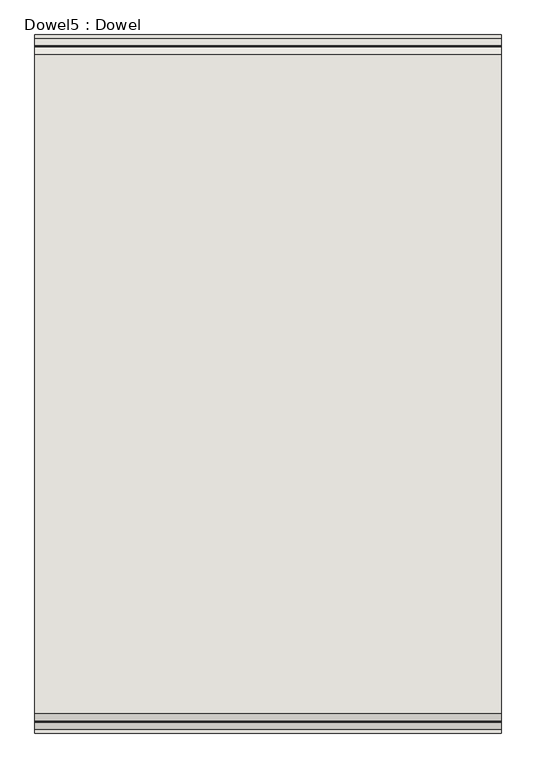
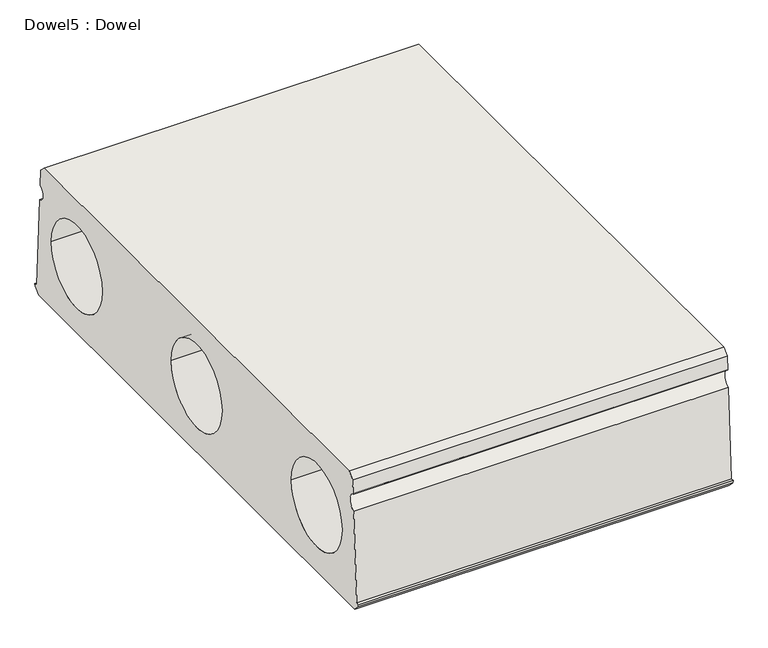
"""IFC4 building model written with IfcOpenShell, lengths in millimetres: wall geometry, Dowel5 : Dowel."""

from ifc_helpers import new_model, si_unit, point, frame, frame_2d, origin, place, context, project, spatial, polyline, circle_curve, trimmed, segment, composite_curve, outline, extrude, source, transform, mapped, element, save


def dowel5_dowel_d00426a0(model_context):
    return source(origin(), model_context, "Body", "SweptSolid", [
        extrude(outline(composite_curve([segment(polyline([(-652.2998095, 2540.0), (494.5752653, 2540.0), (507.2752399, 2527.3000254), (509.1208332, 2491.0485676)]), True, "CONTINUOUS"), segment(trimmed(circle_curve(frame_2d((514.6427832, 2474.6224141)), 17.3294677), [point((509.1208332, 2491.0485676))], [point((511.3260506, 2457.6133067))], True, "CARTESIAN"), True, "CONTINUOUS"), segment(polyline([(511.3260506, 2457.6133067), (523.1502399, 2254.199962), (529.1502279, 2254.199962), (528.4502293, 2248.199974), (515.4502553, 2235.2), (-673.1747995, 2235.2), (-686.1747735, 2248.199974), (-686.8747721, 2254.199962), (-680.8747841, 2254.199962), (-669.0505948, 2457.6133067)]), True, "CONTINUOUS"), segment(trimmed(circle_curve(frame_2d((-675.4772325, 2477.01932)), 20.4424809), [point((-669.0505948, 2457.6133067))], [point((-666.8453774, 2495.55))], True, "CARTESIAN"), True, "CONTINUOUS"), segment(polyline([(-666.8453774, 2495.55), (-664.9997841, 2527.3000254), (-652.2998095, 2540.0)]), True, "CONTINUOUS")], self_intersect=False), holes=[composite_curve([segment(trimmed(circle_curve(frame_2d((-529.7122721, 2387.6)), 95.25), [point((-624.9622721, 2387.6))], [point((-434.4622721, 2387.6))], True, "CARTESIAN"), True, "CONTINUOUS"), segment(trimmed(circle_curve(frame_2d((-529.7122721, 2387.6)), 95.25), [point((-434.4622721, 2387.6))], [point((-624.9622721, 2387.6))], True, "CARTESIAN"), True, "CONTINUOUS")], self_intersect=False), composite_curve([segment(trimmed(circle_curve(frame_2d((-78.8622721, 2387.6)), 95.25), [point((-174.1122721, 2387.6))], [point((16.3877279, 2387.6))], True, "CARTESIAN"), True, "CONTINUOUS"), segment(trimmed(circle_curve(frame_2d((-78.8622721, 2387.6)), 95.25), [point((16.3877279, 2387.6))], [point((-174.1122721, 2387.6))], True, "CARTESIAN"), True, "CONTINUOUS")], self_intersect=False), composite_curve([segment(trimmed(circle_curve(frame_2d((371.9877279, 2387.6)), 95.25), [point((276.7377279, 2387.6))], [point((467.2377279, 2387.6))], True, "CARTESIAN"), True, "CONTINUOUS"), segment(trimmed(circle_curve(frame_2d((371.9877279, 2387.6)), 95.25), [point((467.2377279, 2387.6))], [point((276.7377279, 2387.6))], True, "CARTESIAN"), True, "CONTINUOUS")], self_intersect=False)]), frame((375389.775, 0.0, 0.0), z_axis=(1.0, 0.0, 0.0), x_axis=(0.0, 1.0, 0.0)), (0.0, 0.0, 1.0), 812.8),
    ])


if __name__ == "__main__":
    model = new_model("IFC4")
    model_context = context("Model", 3, world=origin())
    ifc_project = project(units=[si_unit("LENGTHUNIT", "METRE", prefix="MILLI")], contexts=[model_context])
    site = spatial("IfcSite", under=ifc_project)
    building = spatial("IfcBuilding", under=site)
    placement = place(None, origin())
    dowel5_dowel_shape = dowel5_dowel_d00426a0(model_context)
    element("IfcWall", 1, ObjectType="Dowel5 : Dowel", at=placement, inside=building, context=model_context, shape_type="MappedRepresentation", body=[
        mapped(dowel5_dowel_shape, transform((0.0, 0.0, 0.0), x_axis=(1.0, 0.0, 0.0), y_axis=(0.0, 1.0, 0.0), z_axis=(0.0, 0.0, 1.0))),
    ])
    save(model, "model.ifc")

# Revit data of these elements
# Element 1 (IfcWall, "Dowel5 : Dowel")
#   Materials on its faces: "PRECAST PLANK - SEE PRECAST SHOPS FOR SIZE"
# Materials
#   "PRECAST PLANK - SEE PRECAST SHOPS FOR SIZE": class "Concrete", colour RGB 191 191 191, transparency 0, Description = "Cast-in-place concrete", Cost = 0
